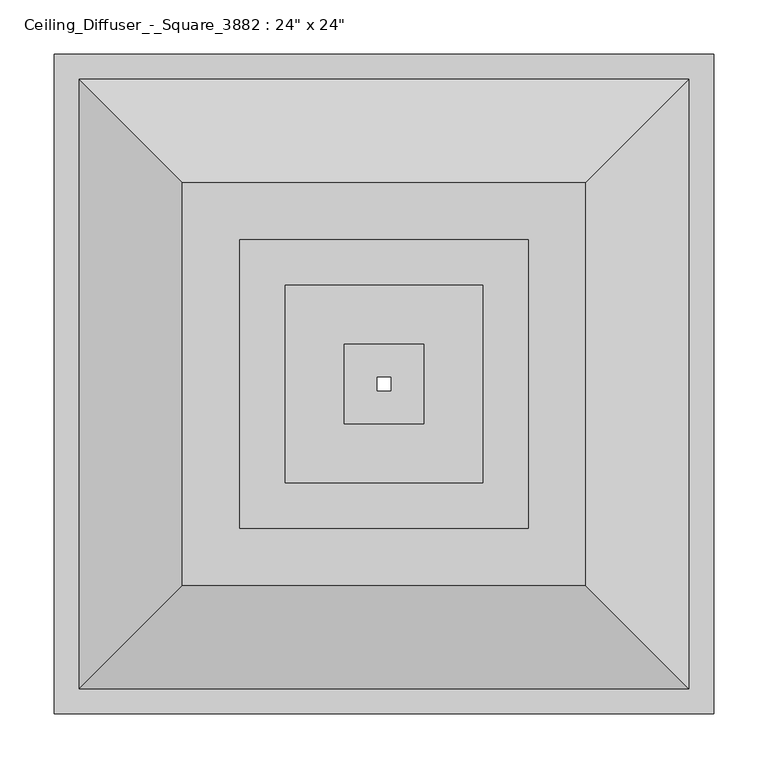
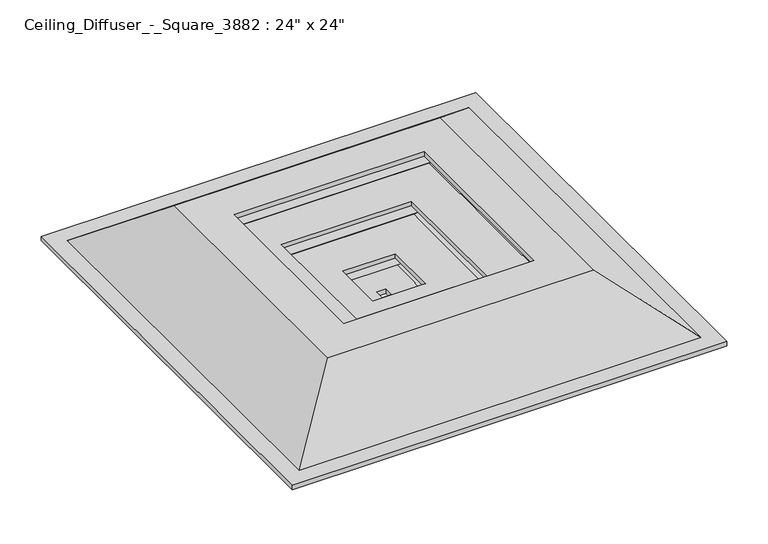
"""IFC4 building model written with IfcOpenShell, lengths in millimetres: proxy geometry."""

from ifc_helpers import new_model, si_unit, origin, place, context, project, spatial, faceted_brep, source, transform, mapped, element, save


def proxy_26d92499(model_context):
    return source(origin(), model_context, "Body", "Brep", [
        faceted_brep([(-76.2, -76.2, 2419.35), (-76.2, -76.2, 2413.0), (76.2, -76.2, 2413.0), (76.2, -76.2, 2419.35), (-43.5024597, -43.5024597, 2432.05), (-59.3774597, -59.3774597, 2419.35), (59.3774597, -59.3774597, 2419.35), (43.5024597, -43.5024597, 2432.05), (-6.35, -6.35, 2425.7), (-6.35, -6.35, 2432.05), (6.35, -6.35, 2432.05), (6.35, -6.35, 2425.7), (-57.15, -57.15, 2413.0), (-41.275, -41.275, 2425.7), (41.275, -41.275, 2425.7), (57.15, -57.15, 2413.0), (76.2, 76.2, 2413.0), (76.2, 76.2, 2419.35), (59.3774597, 59.3774597, 2419.35), (43.5024597, 43.5024597, 2432.05), (6.35, 6.35, 2432.05), (6.35, 6.35, 2425.7), (41.275, 41.275, 2425.7), (57.15, 57.15, 2413.0), (-76.2, 76.2, 2413.0), (-76.2, 76.2, 2419.35), (-59.3774597, 59.3774597, 2419.35), (-43.5024597, 43.5024597, 2432.05), (-6.35, 6.35, 2432.05), (-6.35, 6.35, 2425.7), (-41.275, 41.275, 2425.7), (-57.15, 57.15, 2413.0)], [[[0, 1, 2, 3]], [[4, 5, 6, 7]], [[8, 9, 10, 11]], [[12, 13, 14, 15]], [[3, 2, 16, 17]], [[7, 6, 18, 19]], [[11, 10, 20, 21]], [[15, 14, 22, 23]], [[17, 16, 24, 25]], [[19, 18, 26, 27]], [[21, 20, 28, 29]], [[23, 22, 30, 31]], [[25, 24, 1, 0]], [[3, 17, 25, 0], [5, 26, 18, 6]], [[27, 26, 5, 4]], [[7, 19, 27, 4], [9, 28, 20, 10]], [[29, 28, 9, 8]], [[13, 30, 22, 14], [11, 21, 29, 8]], [[31, 30, 13, 12]], [[1, 24, 16, 2], [15, 23, 31, 12]]]),
        faceted_brep([(-152.4, -152.4, 2425.7), (-152.4, -152.4, 2419.35), (152.4, -152.4, 2419.35), (152.4, -152.4, 2425.7), (-98.1644399, -98.1644399, 2455.6304159), (-135.5774597, -135.5774597, 2425.7), (135.5774597, -135.5774597, 2425.7), (98.1644399, -98.1644399, 2455.6304159), (-36.5125, -36.5125, 2449.2804159), (-36.5125, -36.5125, 2455.6304159), (36.5125, -36.5125, 2455.6304159), (36.5125, -36.5125, 2449.2804159), (-133.35, -133.35, 2419.35), (-95.9369802, -95.9369802, 2449.2804159), (95.9369802, -95.9369802, 2449.2804159), (133.35, -133.35, 2419.35), (152.4, 152.4, 2419.35), (152.4, 152.4, 2425.7), (135.5774597, 135.5774597, 2425.7), (98.1644399, 98.1644399, 2455.6304159), (36.5125, 36.5125, 2455.6304159), (36.5125, 36.5125, 2449.2804159), (95.9369802, 95.9369802, 2449.2804159), (133.35, 133.35, 2419.35), (-152.4, 152.4, 2419.35), (-152.4, 152.4, 2425.7), (-135.5774597, 135.5774597, 2425.7), (-98.1644399, 98.1644399, 2455.6304159), (-36.5125, 36.5125, 2455.6304159), (-36.5125, 36.5125, 2449.2804159), (-95.9369802, 95.9369802, 2449.2804159), (-133.35, 133.35, 2419.35)], [[[0, 1, 2, 3]], [[4, 5, 6, 7]], [[8, 9, 10, 11]], [[12, 13, 14, 15]], [[3, 2, 16, 17]], [[7, 6, 18, 19]], [[11, 10, 20, 21]], [[15, 14, 22, 23]], [[17, 16, 24, 25]], [[19, 18, 26, 27]], [[21, 20, 28, 29]], [[23, 22, 30, 31]], [[25, 24, 1, 0]], [[3, 17, 25, 0], [5, 26, 18, 6]], [[27, 26, 5, 4]], [[7, 19, 27, 4], [9, 28, 20, 10]], [[29, 28, 9, 8]], [[13, 30, 22, 14], [11, 21, 29, 8]], [[31, 30, 13, 12]], [[1, 24, 16, 2], [15, 23, 31, 12]]]),
        faceted_brep([(148.3244802, 148.3244802, 2474.6804159), (209.55, 209.55, 2425.7), (209.55, -209.55, 2425.7), (148.3244802, -148.3244802, 2474.6804159), (91.1744802, 91.1744802, 2481.0304159), (91.1744802, 91.1744802, 2474.6804159), (91.1744802, -91.1744802, 2474.6804159), (91.1744802, -91.1744802, 2481.0304159), (211.7774597, 211.7774597, 2432.05), (150.5519399, 150.5519399, 2481.0304159), (150.5519399, -150.5519399, 2481.0304159), (211.7774597, -211.7774597, 2432.05), (228.6, 228.6, 2425.7), (228.6, 228.6, 2432.05), (228.6, -228.6, 2432.05), (228.6, -228.6, 2425.7), (-209.55, -209.55, 2425.7), (-148.3244802, -148.3244802, 2474.6804159), (-91.1744802, -91.1744802, 2474.6804159), (-91.1744802, -91.1744802, 2481.0304159), (-150.5519399, -150.5519399, 2481.0304159), (-211.7774597, -211.7774597, 2432.05), (-228.6, -228.6, 2432.05), (-228.6, -228.6, 2425.7), (-209.55, 209.55, 2425.7), (-148.3244802, 148.3244802, 2474.6804159), (-91.1744802, 91.1744802, 2474.6804159), (-91.1744802, 91.1744802, 2481.0304159), (-150.5519399, 150.5519399, 2481.0304159), (-211.7774597, 211.7774597, 2432.05), (-228.6, 228.6, 2432.05), (-228.6, 228.6, 2425.7)], [[[0, 1, 2, 3]], [[4, 5, 6, 7]], [[8, 9, 10, 11]], [[12, 13, 14, 15]], [[3, 2, 16, 17]], [[7, 6, 18, 19]], [[11, 10, 20, 21]], [[15, 14, 22, 23]], [[17, 16, 24, 25]], [[19, 18, 26, 27]], [[21, 20, 28, 29]], [[23, 22, 30, 31]], [[15, 23, 31, 12], [1, 24, 16, 2]], [[25, 24, 1, 0]], [[3, 17, 25, 0], [5, 26, 18, 6]], [[27, 26, 5, 4]], [[9, 28, 20, 10], [7, 19, 27, 4]], [[29, 28, 9, 8]], [[13, 30, 22, 14], [11, 21, 29, 8]], [[31, 30, 13, 12]]]),
        faceted_brep([(-184.15, 184.15, 2508.25), (-279.4, 279.4, 2432.05), (279.4, 279.4, 2432.05), (184.15, 184.15, 2508.25), (-133.35, 133.35, 2514.6), (-133.35, 133.35, 2508.25), (133.35, 133.35, 2508.25), (133.35, 133.35, 2514.6), (-281.6274597, 281.6274597, 2438.4), (-186.3774597, 186.3774597, 2514.6), (186.3774597, 186.3774597, 2514.6), (281.6274597, 281.6274597, 2438.4), (-304.8, 304.8, 2432.05), (-304.8, 304.8, 2438.4), (304.8, 304.8, 2438.4), (304.8, 304.8, 2432.05), (279.4, -279.4, 2432.05), (184.15, -184.15, 2508.25), (133.35, -133.35, 2508.25), (133.35, -133.35, 2514.6), (186.3774597, -186.3774597, 2514.6), (281.6274597, -281.6274597, 2438.4), (304.8, -304.8, 2438.4), (304.8, -304.8, 2432.05), (-279.4, -279.4, 2432.05), (-184.15, -184.15, 2508.25), (-133.35, -133.35, 2508.25), (-133.35, -133.35, 2514.6), (-186.3774597, -186.3774597, 2514.6), (-281.6274597, -281.6274597, 2438.4), (-304.8, -304.8, 2438.4), (-304.8, -304.8, 2432.05)], [[[0, 1, 2, 3]], [[4, 5, 6, 7]], [[8, 9, 10, 11]], [[12, 13, 14, 15]], [[3, 2, 16, 17]], [[7, 6, 18, 19]], [[11, 10, 20, 21]], [[15, 14, 22, 23]], [[17, 16, 24, 25]], [[19, 18, 26, 27]], [[21, 20, 28, 29]], [[23, 22, 30, 31]], [[15, 23, 31, 12], [1, 24, 16, 2]], [[25, 24, 1, 0]], [[3, 17, 25, 0], [5, 26, 18, 6]], [[27, 26, 5, 4]], [[9, 28, 20, 10], [7, 19, 27, 4]], [[29, 28, 9, 8]], [[13, 30, 22, 14], [11, 21, 29, 8]], [[31, 30, 13, 12]]]),
    ])


if __name__ == "__main__":
    model = new_model("IFC4")
    model_context = context("Model", 3, world=origin())
    ifc_project = project(units=[si_unit("LENGTHUNIT", "METRE", prefix="MILLI")], contexts=[model_context])
    site = spatial("IfcSite", under=ifc_project)
    building = spatial("IfcBuilding", under=site)
    placement = place(None, origin())
    proxy_shape = proxy_26d92499(model_context)
    element("IfcBuildingElementProxy", 1, Name="Ceiling_Diffuser_-_Square_3882 : 24\" x 24\"", ObjectType="Ceiling_Diffuser_-_Square_3882 : 24\" x 24\"", at=placement, inside=building, context=model_context, shape_type="MappedRepresentation", body=[
        mapped(proxy_shape, transform((0.0, 0.0, 0.0), x_axis=(1.0, 0.0, 0.0), y_axis=(0.0, 1.0, 0.0), z_axis=(0.0, 0.0, 1.0))),
    ])
    save(model, "model.ifc")

# Revit data of these elements
# Type "Ceiling_Diffuser_-_Square_3882 : 24\" x 24\""
#   Width = 2' - 0"
#   Length = 2' - 0"
#   Diffuser Finish = none
